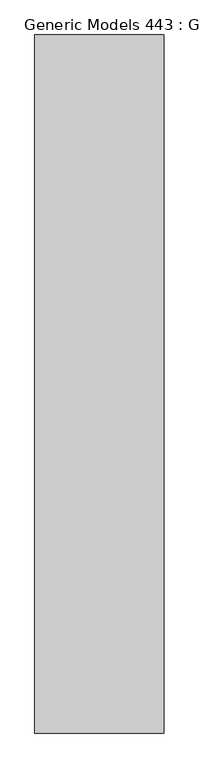
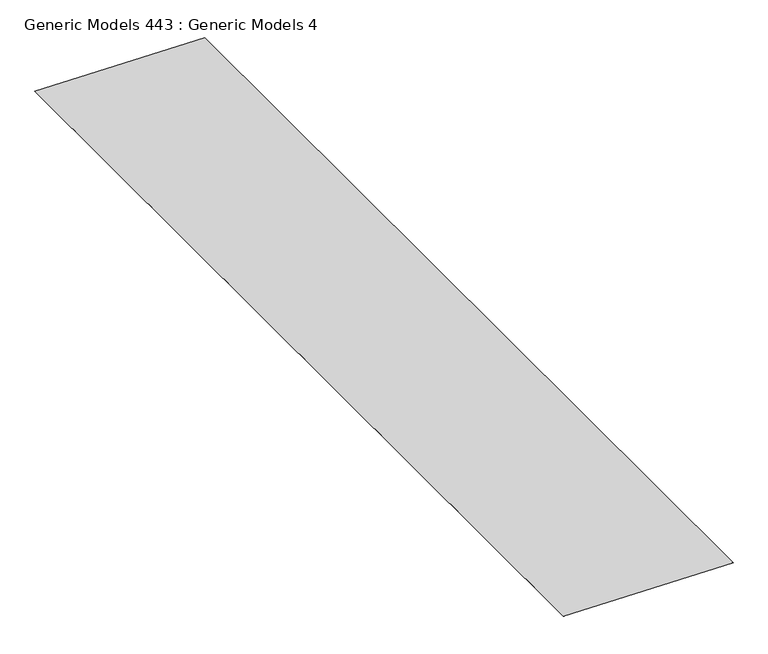
"""IFC4 building model written with IfcOpenShell, lengths in millimetres: proxy geometry, Generic Models 443 : Generic Models 4."""

from ifc_helpers import new_model, si_unit, frame, origin, place, context, project, spatial, polyline, outline, extrude, source, transform, mapped, element, save


def generic_models_443_generic_models_4_957b986e(model_context):
    return source(origin(), model_context, "Body", "SweptSolid", [
        extrude(outline(polyline([(126757.0052644, -8159.3046574), (126732.6548985, -6764.2731291), (126733.4487694, -6764.2731291), (126757.7988935, -8159.2908046), (126757.0052644, -8159.3046574)])), frame((0.0, -464.1230338, 0.0), z_axis=(0.0, 1.0, 0.0), x_axis=(0.0, 0.0, 1.0)), (0.0, 0.0, 1.0), 7518.4),
    ])


if __name__ == "__main__":
    model = new_model("IFC4")
    model_context = context("Model", 3, world=origin())
    ifc_project = project(units=[si_unit("LENGTHUNIT", "METRE", prefix="MILLI")], contexts=[model_context])
    site = spatial("IfcSite", under=ifc_project)
    building = spatial("IfcBuilding", under=site)
    placement = place(None, origin())
    generic_models_443_generic_models_4_shape = generic_models_443_generic_models_4_957b986e(model_context)
    element("IfcBuildingElementProxy", 1, Name="Generic Models 443 : Generic Models 4", ObjectType="Generic Models 443 : Generic Models 4", at=placement, inside=building, context=model_context, shape_type="MappedRepresentation", body=[
        mapped(generic_models_443_generic_models_4_shape, transform((0.0, 0.0, 0.0), x_axis=(1.0, 0.0, 0.0), y_axis=(0.0, 1.0, 0.0), z_axis=(0.0, 0.0, 1.0))),
    ])
    save(model, "model.ifc")

# Revit data of these elements
# Element 1 (IfcBuildingElementProxy, "Generic Models 443 : Generic Models 4")
#   Materials on its faces: "_SEPERATION MEMBRANE UNDER EACH SLEEPER"
# Materials
#   "_SEPERATION MEMBRANE UNDER EACH SLEEPER": class "Generic", colour RGB 253 192 103, transparency 0, Cost = 0
